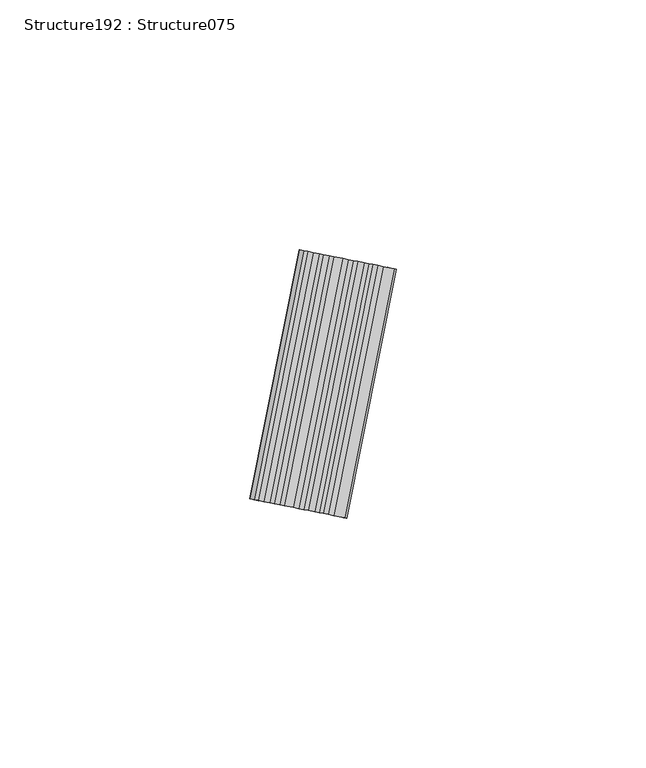
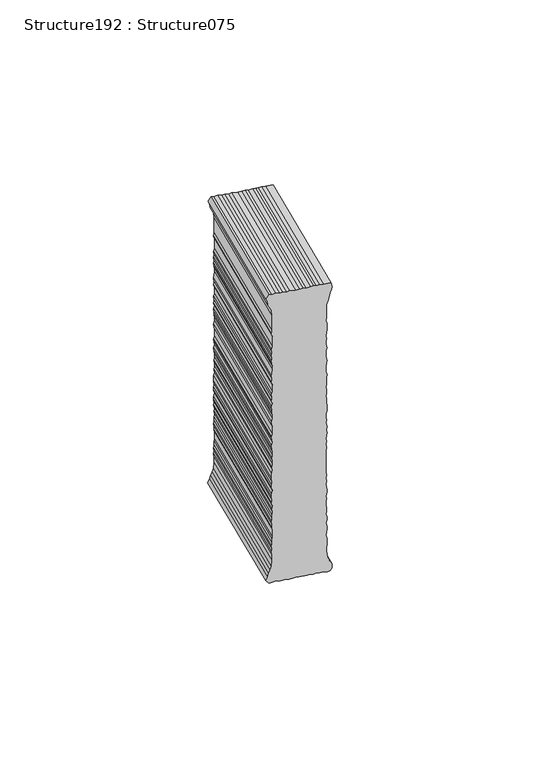
"""IFC4 building model written with IfcOpenShell, lengths in millimetres: proxy geometry, Structure192 : Structure075."""

from ifc_helpers import new_model, si_unit, frame, origin, place, context, project, spatial, polyline, outline, extrude, source, transform, mapped, element, save


def structure192_structure075_4603cae3(model_context):
    return source(origin(), model_context, "Body", "SweptSolid", [
        extrude(outline(polyline([(1.8233335, 0.0), (3.1470297, 0.293028), (4.2244865, 0.7376621), (5.4061289, 0.9114746), (6.4793271, 1.3564169), (7.453505, 0.374405), (7.3876839, -0.5348157), (7.0413299, -1.6823692), (7.2469213, -2.4792418), (7.1626024, -3.6439811), (6.9587855, -4.6705705), (7.0218141, -5.5887622), (6.8180229, -6.6149967), (6.6191448, -7.5142283), (6.677363, -8.5580033), (6.5082886, -10.8935151), (6.3003415, -11.9180217), (6.5059586, -12.7145394), (6.1595789, -13.8624479), (6.2363462, -14.6499946), (6.1423932, -15.9478165), (6.1963785, -16.9909285), (6.0112391, -17.759515), (5.0532803, -18.342299), (3.7708431, -18.1196038), (2.7725399, -17.5250562), (1.8899032, -17.0723054), (1.0114786, -16.6155787), (-1.0399, -16.2077184), (-2.0754605, -16.1327512), (-3.1246312, -16.1866546), (-5.1943325, -16.036823), (-6.3503054, -15.6934271), (-7.5226219, -15.7384155), (-8.43871, -15.8019531), (-9.3454464, -15.7363119), (-10.6227907, -15.3841296), (-11.6774093, -15.5674944), (-12.7168735, -15.4922446), (-13.5992284, -15.1686567), (-14.5213496, -15.2317575), (-15.6843145, -15.1475671), (-16.7108781, -14.9433954), (-17.7503424, -14.8681456), (-18.7938348, -14.92246), (-19.9492226, -14.7089623), (-21.0077449, -14.8920445), (-21.9144813, -14.8264033), (-22.8118661, -14.6315831), (-23.8366554, -14.4275399), (-24.8819223, -14.4817258), (-26.0451176, -14.2676629), (-26.9573018, -14.3314831), (-28.1165932, -14.1177028), (-35.504632, -13.5828614), (-36.2915412, -13.6557507), (-37.5800115, -13.4326187), (-38.6231492, -13.4869589), (-39.3938393, -13.3013105), (-40.5661558, -13.346299), (-41.4822438, -13.4098366), (-42.5127113, -13.2053823), (-43.6850278, -13.2503708), (-44.8310639, -12.9076942), (-45.7510557, -12.9709492), (-46.904669, -12.75758), (-47.9441332, -12.6823302), (-48.9987517, -12.865695), (-50.9453073, -12.7247782), (-51.8391432, -12.530215), (-53.1348358, -12.4364161), (-54.0325755, -12.2415703), (-55.2105702, -12.2861477), (-56.244711, -12.2112833), (-57.1420959, -12.0164632), (-58.057829, -12.0800264), (-60.395825, -11.9107722), (-61.4347039, -11.9654206), (-62.4561747, -11.6317617), (-64.2753257, -11.5000681), (-65.4479971, -11.5450309), (-66.358407, -11.6089796), (-67.514025, -11.2656094), (-69.5837263, -11.1157777), (-70.5095209, -11.3084685), (-71.7865103, -10.9563119), (-72.8220707, -10.8813447), (-73.6093348, -10.9542082), (-74.7633029, -10.7408133), (-75.814248, -10.7945882), (-76.7303361, -10.8581258), (-78.9327652, -10.6986856), (-79.8207983, -10.3746866), (-80.9987931, -10.419264), (-85.2712784, -10.1099665), (-87.1286228, -10.4960017), (-88.4487235, -10.793571), (-89.368916, -10.854671), (-90.3000349, -11.180043), (-91.3524984, -11.3632072), (-92.6260665, -10.8800153), (-92.4666006, -8.6772313), (-92.5113322, -7.5013659), (-92.307032, -6.4730278), (-92.3799983, -5.6871833), (-92.3142543, -4.7790273), (-91.9643553, -3.5036582), (-92.1549168, -2.5780178), (-91.950591, -1.5493248), (-91.7392225, -0.393783), (-91.86404, 1.4400135), (-91.5421703, 2.3282008), (-91.7139001, 3.5139735), (-91.5191057, 4.4110033), (-91.5637858, 5.5875785), (-91.2230844, 6.735898), (-91.4229975, 7.5323596), (-89.9359318, 8.2045553), (-89.1900807, 7.7595664), (-87.9038939, 7.5344593), (-85.9090056, 6.3511965), (-83.842777, 6.0696199), (-78.9197837, 5.7132303), (-77.74128, 5.7599114), (-76.8537302, 5.4341636), (-73.4823032, 5.1900963), (-72.4272012, 5.3752099), (-71.4032759, 5.1690886), (-70.4866788, 5.2347299), (-69.3275415, 5.0188203), (-68.4109444, 5.0844615), (-67.3845349, 4.8781604), (-66.4867694, 4.6836695), (-65.4473053, 4.6084197), (-63.3587722, 4.7187202), (-62.199635, 4.5028106), (-61.0268094, 4.5499027), (-60.1335814, 4.2237439), (-57.9364757, 4.0646891), (-57.137957, 4.2683775), (-55.8517702, 4.0432704), (-54.8059941, 4.09956), (-53.9145406, 3.7735296), (-52.8597935, 3.958669), (-51.7063344, 3.7431704), (-50.799598, 3.6775291), (-49.7726538, 3.4736865), (-48.7331896, 3.3984367), (-47.5457148, 3.5739675), (-45.7507187, 3.1825271), (-43.4191107, 3.0137353), (-42.3664931, 3.1990287), (-41.5959571, 3.0112511), (-40.565464, 2.8071516), (-39.5128462, 2.992445), (-38.2305631, 2.7676205), (-37.20007, 2.563521), (-36.1641547, 2.4885281), (-35.1189134, 2.5423592), (-34.0887752, 2.3382854), (-33.0546342, 2.263421), (-32.0058441, 2.3169952), (-30.9792548, 2.1131783), (-29.9245077, 2.2983176), (-28.11068, 2.1670094), (-26.9533171, 1.9512282), (-26.0370749, 2.0168952), (-24.8723356, 1.9325763), (-23.9805271, 1.6065203), (-22.7987305, 1.7824621), (-21.7628152, 1.7074692), (-20.8595515, 1.510083), (-19.8162597, 1.5665524), (-18.6664484, 1.2218188), (-17.750031, 1.2849758), (-16.7234417, 1.081159), (-15.6803297, 1.1351442), (-14.3846372, 1.0413453), (-13.46804, 1.1069865), (-12.4359523, 0.9002744), (-11.2729874, 0.816084), (-10.5047558, 0.6309704), (-8.1727929, 0.4621529), (-7.3837802, 0.5345331), (-6.0880875, 0.4407342), (-5.0426664, 0.4970495), (-4.0123531, 0.2904658), (-3.2288387, 0.3657413), (-1.9426518, 0.1406342), (0.0, 0.0), (1.8233335, 0.0)])), frame((-2007.9452541, 234866.9720294, 393.8064615), z_axis=(0.19466222296394123, 0.9808703374813295, 0.0), x_axis=(-0.07082268804927393, 0.01405537650098564, -0.9973898902880913)), (0.0, 0.0, 1.0), 50.8),
    ])


if __name__ == "__main__":
    model = new_model("IFC4")
    model_context = context("Model", 3, world=origin())
    ifc_project = project(units=[si_unit("LENGTHUNIT", "METRE", prefix="MILLI")], contexts=[model_context])
    site = spatial("IfcSite", under=ifc_project)
    building = spatial("IfcBuilding", under=site)
    placement = place(None, origin())
    structure192_structure075_shape = structure192_structure075_4603cae3(model_context)
    element("IfcBuildingElementProxy", 1, Name="Structure192 : Structure075", ObjectType="Structure192 : Structure075", at=placement, inside=building, context=model_context, shape_type="MappedRepresentation", body=[
        mapped(structure192_structure075_shape, transform((0.0, 0.0, 0.0), x_axis=(1.0, 0.0, 0.0), y_axis=(0.0, 1.0, 0.0), z_axis=(0.0, 0.0, 1.0))),
    ])
    save(model, "model.ifc")

# Revit data of these elements
# Type "Structure192 : Structure075"
#   NameOverride = "Structure075"
# Element 1 (IfcBuildingElementProxy, "Structure192 : Structure075")
#   Materials on its faces: "BRUSHED ALUMINUM LETTERING"
# Materials
#   "BRUSHED ALUMINUM LETTERING": class "Unassigned", colour RGB 169 181 186, transparency 0, Cost = 0
